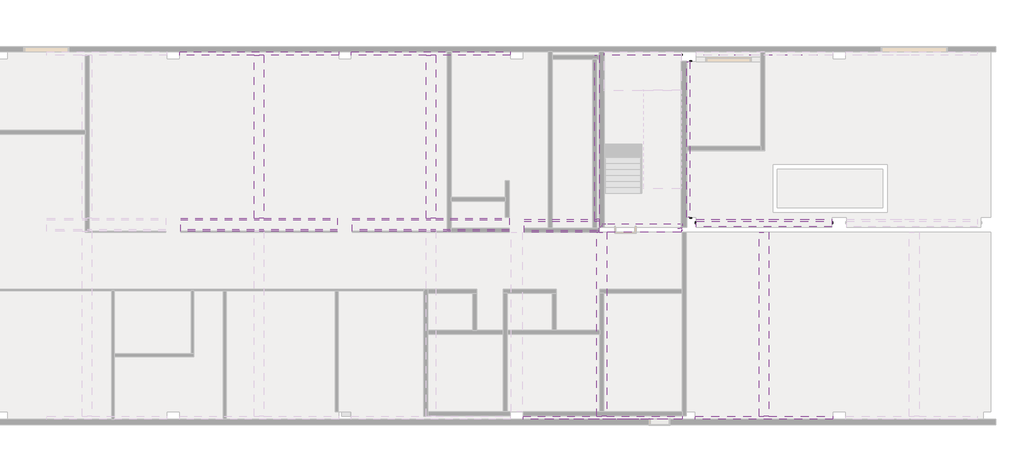
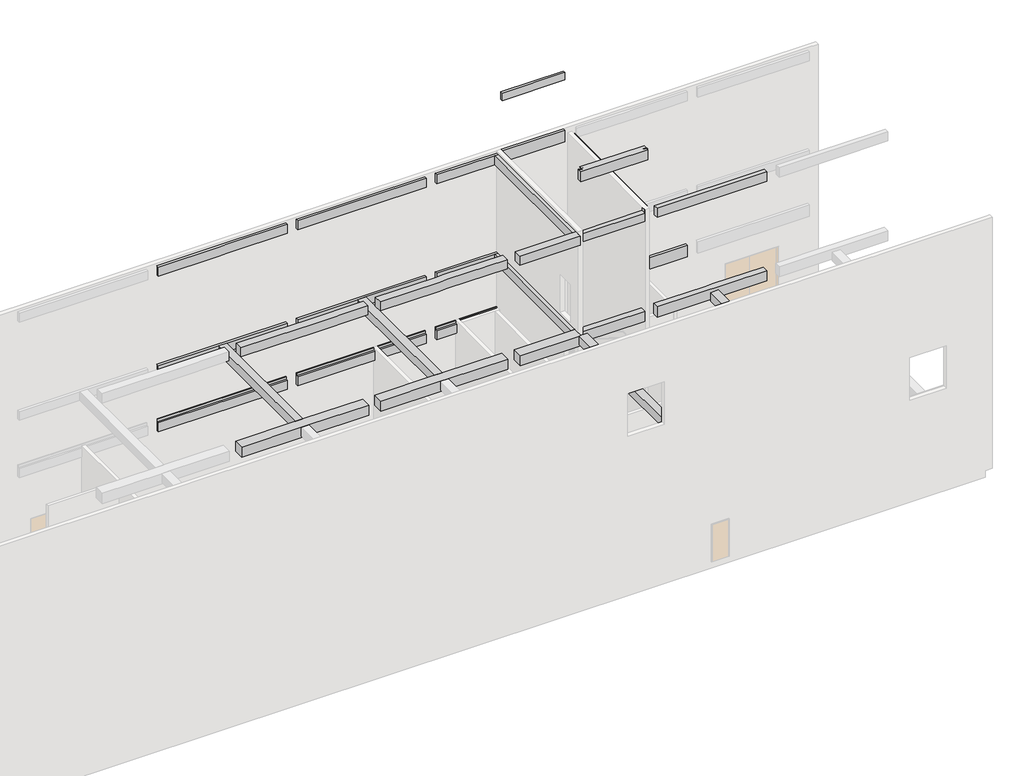
# One storey, part 4 of 5: 55 beams.
"""IFC4 building model written with IfcOpenShell, lengths in millimetres."""

from ifc_helpers import new_model, si_unit, frame, origin, place, context, project, spatial, polyline, outline, extrude, faceted_brep, element, save

model = new_model("IFC4")

# Units and contexts
model_context = context("Model", 3, world=origin())
ifc_project = project(units=[si_unit("LENGTHUNIT", "METRE", prefix="MILLI")], contexts=[model_context])

# Site, building, storey
site = spatial("IfcSite", under=ifc_project)
building = spatial("IfcBuilding", under=site)
storey = spatial("IfcBuildingStorey", under=building, Name="TOC", Elevation=149.9618634)

# Beams
placement = place(None, origin())
element("IfcBeam", 1, ObjectType="RC Beam_Rectangular : H_SB_AR_S16_UG_B500xH700_1G1", at=placement, inside=storey, context=model_context, shape_type="Brep", body=[
    faceted_brep([(61750.0, 799.5208589, -0.0381366), (61750.0, 9149.5208589, -0.0381366), (61750.0, 9149.5208589, -150.0381366), (61750.0, 9149.5208589, -550.0381366), (61750.0, 799.5208589, -550.0381366), (62250.0, 9149.5208589, -550.0381366), (62250.0, 799.5208589, -550.0381366), (62250.0, 9149.5208589, -0.0381366), (62250.0, 799.5208589, -0.0381366), (62250.0, 9149.5208589, -150.0381366)], [[[0, 1, 2, 3, 4]], [[3, 5, 6, 4]], [[7, 8, 6, 5, 9]], [[1, 0, 8, 7]], [[5, 3, 2, 1, 7, 9]], [[4, 6, 8, 0]]]),
])
element("IfcBeam", 2, ObjectType="RC Beam_Rectangular : H_SB_AR_S16_UG_B500xH700_1G1", at=placement, inside=storey, context=model_context, shape_type="Brep", body=[
    faceted_brep([(54700.0, 799.5208589, -0.0381366), (54700.0, 9149.5208589, -0.0381366), (54700.0, 9149.5208589, -150.0381366), (54700.0, 9149.5208589, -550.0381366), (54700.0, 799.5208589, -550.0381366), (54700.0, 799.5208589, -150.0381366), (55200.0, 799.5208589, -550.0381366), (54850.0, 9149.5208589, -550.0381366), (55200.0, 9149.5208589, -550.0381366), (55200.0, 9149.5208589, -0.0381366), (55200.0, 799.5208589, -0.0381366), (55200.0, 9149.5208589, -150.0381366)], [[[0, 1, 2, 3, 4, 5]], [[6, 4, 3, 7, 8]], [[9, 10, 6, 8, 11]], [[1, 0, 10, 9]], [[1, 9, 11, 8, 7, 3, 2]], [[4, 6, 10, 0, 5]]]),
])
element("IfcBeam", 3, ObjectType="RC Beam_Rectangular : H_SB_AR_S16_UG_B450xH700_1B2", at=placement, inside=storey, context=model_context, shape_type="SweptSolid", body=[
    extrude(outline(polyline([(57725.0, 599.5208589), (57275.0, 599.5208589), (57275.0, 9149.5208589), (57725.0, 9149.5208589), (57725.0, 599.5208589)])), frame((0.0, 0.0, -550.0381366), z_axis=(0.0, 0.0, 1.0), x_axis=(1.0, 0.0, 0.0)), (0.0, 0.0, 1.0), 550.0),
])
element("IfcBeam", 4, ObjectType="RC Beam_Rectangular : H_SB_AR_S16_UG_B450xH700_1B2", at=placement, inside=storey, context=model_context, shape_type="SweptSolid", body=[
    extrude(outline(polyline([(60225.0, 599.5208589), (59775.0, 599.5208589), (59775.0, 9149.5208589), (60225.0, 9149.5208589), (60225.0, 599.5208589)])), frame((0.0, 0.0, -550.0381366), z_axis=(0.0, 0.0, 1.0), x_axis=(1.0, 0.0, 0.0)), (0.0, 0.0, 1.0), 550.0),
])
element("IfcBeam", 5, ObjectType="RC Beam_Rectangular : H_SB_AR_S16_UG_B450xH700_1B1A", at=placement, inside=storey, context=model_context, shape_type="Brep", body=[
    faceted_brep([(51175.0, 599.5208589, -0.0381366), (51175.0, 599.5208589, -550.0381366), (51175.0, 9149.5208589, -550.0381366), (51175.0, 9149.5208589, -0.0381366), (50725.0, 599.5208589, -550.0381366), (50725.0, 9199.5208589, -550.0381366), (50725.0, 9799.5208589, -550.0381366), (50825.0, 9799.5208589, -550.0381366), (50825.0, 9149.5208589, -550.0381366), (50725.0, 599.5208589, -0.0381366), (50725.0, 9199.5208589, -0.0381366), (50725.0, 9799.5208589, -0.0381366), (50825.0, 9149.5208589, -0.0381366), (50825.0, 9799.5208589, -0.0381366)], [[[0, 1, 2, 3]], [[4, 5, 6, 7, 8, 2, 1]], [[6, 5, 4, 9, 10, 11]], [[4, 1, 0, 9]], [[0, 3, 12, 13, 11, 10, 9]], [[12, 8, 7, 13]], [[6, 11, 13, 7]], [[8, 12, 3, 2]]]),
])
element("IfcBeam", 6, ObjectType="RC Beam_Rectangular : H_SB_AR_S16_UG_B500xH700_1G3", at=placement, inside=storey, context=model_context, shape_type="SweptSolid", body=[
    extrude(outline(polyline([(-550.0381366, 55300.0), (-550.0381366, 61700.0), (-150.0381366, 61700.0), (-150.0381366, 61650.0), (-0.0381366, 61650.0), (-0.0381366, 55350.0), (-150.0381366, 55350.0), (-150.0381366, 55300.0), (-550.0381366, 55300.0)])), frame((0.0, 9549.5208589, 0.0), z_axis=(0.0, 1.0, 0.0), x_axis=(0.0, 0.0, 1.0)), (0.0, 0.0, 1.0), 100.0),
])
element("IfcBeam", 7, ObjectType="RC Beam_Rectangular : H_SB_AR_S16_UG_B600xH800_1G2", at=placement, inside=storey, context=model_context, shape_type="SweptSolid", body=[
    extrude(outline(polyline([(51225.0, 9799.5208589), (54650.0, 9799.5208589), (54650.0, 9549.5208589), (51225.0, 9549.5208589), (51225.0, 9799.5208589)])), frame((0.0, 0.0, -550.0381366), z_axis=(0.0, 0.0, 1.0), x_axis=(1.0, 0.0, 0.0)), (0.0, 0.0, 1.0), 500.0),
    extrude(outline(polyline([(-150.0381366, 47300.0), (-550.0381366, 47300.0), (-550.0381366, 48250.0), (-650.0381366, 48250.0), (-650.0381366, 49775.0), (-550.0381366, 49775.0), (-550.0381366, 50725.0), (-0.0381366, 50725.0), (-0.0381366, 47350.0), (-150.0381366, 47350.0), (-150.0381366, 47300.0)])), frame((0.0, 9199.5208589, 0.0), z_axis=(0.0, 1.0, 0.0), x_axis=(0.0, 0.0, 1.0)), (0.0, 0.0, 1.0), 600.0),
])
element("IfcBeam", 8, ObjectType="RC Beam_Rectangular : H_SB_AR_S16_UG_B600xH800_1G2", at=placement, inside=storey, context=model_context, shape_type="Brep", body=[
    faceted_brep([(39300.0, 9749.5208589, -550.0381366), (39300.0, 9749.5208589, -150.0381366), (39350.0, 9749.5208589, -150.0381366), (39350.0, 9749.5208589, -0.0381366), (42775.0, 9749.5208589, -0.0381366), (43225.0, 9749.5208589, -0.0381366), (46650.0, 9749.5208589, -0.0381366), (46650.0, 9749.5208589, -150.0381366), (46700.0, 9749.5208589, -150.0381366), (46700.0, 9749.5208589, -550.0381366), (45750.0, 9749.5208589, -550.0381366), (45750.0, 9749.5208589, -650.0381366), (40250.0, 9749.5208589, -650.0381366), (40250.0, 9749.5208589, -550.0381366), (40250.0, 9149.5208589, -650.0381366), (45750.0, 9149.5208589, -650.0381366), (38750.0, 9149.5208589, -550.0381366), (40250.0, 9149.5208589, -550.0381366), (45750.0, 9149.5208589, -550.0381366), (46750.0, 9149.5208589, -550.0381366), (47250.0, 9149.5208589, -550.0381366), (47250.0, 9149.5208589, -150.0381366), (46650.0, 9149.5208589, -150.0381366), (46650.0, 9149.5208589, -0.0381366), (43225.0, 9149.5208589, -0.0381366), (42775.0, 9149.5208589, -0.0381366), (39350.0, 9149.5208589, -0.0381366), (39350.0, 9149.5208589, -150.0381366), (38750.0, 9149.5208589, -150.0381366), (39300.0, 9199.5208589, -550.0381366), (39300.0, 9199.5208589, -150.0381366), (46700.0, 9199.5208589, -150.0381366), (46700.0, 9199.5208589, -550.0381366), (38750.0, 9199.5208589, -550.0381366), (46750.0, 9199.5208589, -550.0381366), (47250.0, 9199.5208589, -550.0381366), (38750.0, 9199.5208589, -150.0381366), (46750.0, 9199.5208589, -150.0381366), (47250.0, 9199.5208589, -150.0381366)], [[[0, 1, 2, 3, 4, 5, 6, 7, 8, 9, 10, 11, 12, 13]], [[14, 12, 11, 15]], [[16, 17, 14, 15, 18, 19, 20, 21, 22, 23, 24, 25, 26, 27, 28]], [[29, 30, 1, 0]], [[31, 32, 9, 8]], [[13, 17, 16, 33, 29, 0]], [[17, 13, 12, 14]], [[18, 10, 9, 32, 34, 35, 20, 19]], [[10, 18, 15, 11]], [[3, 26, 25, 24, 23, 6, 5, 4]], [[30, 29, 33, 36]], [[32, 31, 37, 38, 35, 34]], [[27, 2, 1, 30, 36, 28]], [[2, 27, 26, 3]], [[7, 22, 21, 38, 37, 31, 8]], [[22, 7, 6, 23]], [[36, 33, 16, 28]], [[20, 35, 38, 21]]]),
])
element("IfcBeam", 9, ObjectType="RC Beam_Rectangular : H_SB_AR_S16_UG_B600xH800_1G2", at=placement, inside=storey, context=model_context, shape_type="Brep", body=[
    faceted_brep([(38700.0, 9749.5208589, -150.0381366), (38700.0, 9749.5208589, -550.0381366), (37797.3745649, 9749.5208589, -550.0381366), (37797.3745649, 9749.5208589, -0.0381366), (38650.0, 9749.5208589, -0.0381366), (38650.0, 9749.5208589, -150.0381366), (37797.3745649, 9500.8571094, -550.0381366), (37797.3745649, 9500.8571094, -0.0381366), (38650.0, 9499.9097478, -0.0381366), (38650.0, 9499.9097478, -150.0381366), (38700.0, 9499.8541922, -150.0381366), (38700.0, 9499.8541922, -550.0381366)], [[[0, 1, 2, 3, 4, 5]], [[2, 6, 7, 3]], [[3, 7, 8, 4]], [[5, 9, 10, 0]], [[11, 10, 9, 8, 7, 6]], [[1, 0, 10, 11]], [[2, 1, 11, 6]], [[9, 5, 4, 8]]]),
    faceted_brep([(38749.6109568, 9149.5208589, -150.0381366), (38749.6109568, 9149.5208589, -550.0381366), (38750.0, 9149.5208589, -550.0381366), (38750.0, 9149.5208589, -150.0381366), (38749.6665123, 9199.5208589, -550.0381366), (38750.0, 9199.5208589, -550.0381366), (38749.6665123, 9199.5208589, -150.0381366), (38750.0, 9199.5208589, -150.0381366)], [[[0, 1, 2, 3]], [[1, 4, 5, 2]], [[4, 6, 7, 5]], [[6, 4, 1, 0]], [[3, 2, 5, 7]], [[6, 0, 3, 7]]]),
])
element("IfcBeam", 10, ObjectType="RC Beam_Rectangular : H_SB_AR_S16_UG_B450xH700_1B1", at=placement, inside=storey, context=model_context, shape_type="SweptSolid", body=[
    extrude(outline(polyline([(34775.0, 17399.5208589), (35225.0, 17399.5208589), (35225.0, 9749.5208589), (34775.0, 9749.5208589), (34775.0, 17399.5208589)])), frame((0.0, 0.0, -550.0381366), z_axis=(0.0, 0.0, 1.0), x_axis=(1.0, 0.0, 0.0)), (0.0, 0.0, 1.0), 550.0),
])
element("IfcBeam", 11, ObjectType="RC Beam_Rectangular : H_SB_AR_S16_UG_B450xH700_1B1", at=placement, inside=storey, context=model_context, shape_type="SweptSolid", body=[
    extrude(outline(polyline([(42775.0, 17399.5208589), (43225.0, 17399.5208589), (43225.0, 9749.5208589), (42775.0, 9749.5208589), (42775.0, 17399.5208589)])), frame((0.0, 0.0, -550.0381366), z_axis=(0.0, 0.0, 1.0), x_axis=(1.0, 0.0, 0.0)), (0.0, 0.0, 1.0), 550.0),
])
element("IfcBeam", 12, ObjectType="RC Beam_Rectangular : H_SB_AR_S16_UG_B500xH700_1G1", at=placement, inside=storey, context=model_context, shape_type="SweptSolid", body=[
    extrude(outline(polyline([(17199.5208589, -550.0381366), (9799.5208589, -550.0381366), (9799.5208589, -150.0381366), (9849.5208589, -150.0381366), (9849.5208589, -0.0381366), (17199.5208589, -0.0381366), (17199.5208589, -550.0381366)])), frame((46750.0, 0.0, 0.0), z_axis=(1.0, 0.0, 0.0), x_axis=(0.0, 1.0, 0.0)), (0.0, 0.0, 1.0), 500.0),
])
element("IfcBeam", 13, ObjectType="RC Beam_Rectangular : H_SB_AR_S16_UG_B500xH700_1G1", at=placement, inside=storey, context=model_context, shape_type="SweptSolid", body=[
    extrude(outline(polyline([(9799.5208589, -550.0381366), (9799.5208589, -150.0381366), (9849.5208589, -150.0381366), (9849.5208589, -0.0381366), (17199.5208589, -0.0381366), (17199.5208589, -550.0381366), (9799.5208589, -550.0381366)])), frame((38750.0, 0.0, 0.0), z_axis=(1.0, 0.0, 0.0), x_axis=(0.0, 1.0, 0.0)), (0.0, 0.0, 1.0), 500.0),
])
element("IfcBeam", 14, ObjectType="RC Beam_Rectangular : H_SB_AR_S16_UG_B500xH700_1G1", at=placement, inside=storey, context=model_context, shape_type="SweptSolid", body=[
    extrude(outline(polyline([(17149.5208589, -550.0381366), (9799.5208589, -550.0381366), (9799.5208589, -150.0381366), (9849.5208589, -150.0381366), (9849.5208589, -0.0381366), (17099.5208589, -0.0381366), (17099.5208589, -150.0381366), (17149.5208589, -150.0381366), (17149.5208589, -550.0381366)])), frame((55050.0, 0.0, 0.0), z_axis=(1.0, 0.0, 0.0), x_axis=(0.0, 1.0, 0.0)), (0.0, 0.0, 1.0), 100.0),
    extrude(outline(polyline([(54650.0, 17449.5208589), (54700.0, 17449.5208589), (54700.0, 17399.5208589), (54650.0, 17399.5208589), (54650.0, 17449.5208589)])), frame((0.0, 0.0, -550.0381366), z_axis=(0.0, 0.0, 1.0), x_axis=(1.0, 0.0, 0.0)), (0.0, 0.0, 1.0), 400.0),
])
element("IfcBeam", 15, ObjectType="RC Beam_Rectangular : H_SB_AR_S16_AG_B400xH700_3WG1", at=placement, inside=storey, context=model_context, shape_type="Brep", body=[
    faceted_brep([(31300.0, 17499.5208589, 5949.9618634), (38700.0, 17499.5208589, 5949.9618634), (38700.0, 17549.5208589, 5949.9618634), (31300.0, 17549.5208589, 5949.9618634), (31300.0, 17399.5208589, 5799.9618634), (31300.0, 17399.5208589, 5249.9618634), (34775.0, 17399.5208589, 5249.9618634), (35225.0, 17399.5208589, 5249.9618634), (38700.0, 17399.5208589, 5249.9618634), (38700.0, 17399.5208589, 5799.9618634), (35225.0, 17399.5208589, 5799.9618634), (34775.0, 17399.5208589, 5799.9618634), (31300.0, 17549.5208589, 5249.9618634), (38700.0, 17549.5208589, 5249.9618634), (31300.0, 17499.5208589, 5799.9618634), (38700.0, 17499.5208589, 5799.9618634)], [[[0, 1, 2, 3]], [[4, 5, 6, 7, 8, 9, 10, 11]], [[8, 7, 6, 5, 12, 13]], [[14, 4, 11, 10, 9, 15]], [[0, 14, 15, 1]], [[5, 4, 14, 0, 3, 12]], [[9, 8, 13, 2, 1, 15]], [[3, 2, 13, 12]]]),
])
element("IfcBeam", 16, ObjectType="RC Beam_Rectangular : H_SB_AR_S16_AG_B400xH700_3WG1", at=placement, inside=storey, context=model_context, shape_type="Brep", body=[
    faceted_brep([(39300.0, 17499.5208589, 5949.9618634), (46700.0, 17499.5208589, 5949.9618634), (46700.0, 17549.5208589, 5949.9618634), (39300.0, 17549.5208589, 5949.9618634), (39300.0, 17399.5208589, 5799.9618634), (39300.0, 17399.5208589, 5249.9618634), (42775.0, 17399.5208589, 5249.9618634), (43225.0, 17399.5208589, 5249.9618634), (46700.0, 17399.5208589, 5249.9618634), (46700.0, 17399.5208589, 5799.9618634), (43225.0, 17399.5208589, 5799.9618634), (42775.0, 17399.5208589, 5799.9618634), (39300.0, 17549.5208589, 5249.9618634), (46700.0, 17549.5208589, 5249.9618634), (39300.0, 17499.5208589, 5799.9618634), (46700.0, 17499.5208589, 5799.9618634)], [[[0, 1, 2, 3]], [[4, 5, 6, 7, 8, 9, 10, 11]], [[8, 7, 6, 5, 12, 13]], [[14, 4, 11, 10, 9, 15]], [[0, 14, 15, 1]], [[5, 4, 14, 0, 3, 12]], [[9, 8, 13, 2, 1, 15]], [[3, 2, 13, 12]]]),
])
element("IfcBeam", 17, ObjectType="RC Beam_Rectangular : H_SB_AR_S16_AG_B400xH700_3WG1", at=placement, inside=storey, context=model_context, shape_type="Brep", body=[
    faceted_brep([(51075.0, 17549.5208589, 5949.9618634), (51075.0, 17399.5208589, 5949.9618634), (54650.0, 17399.5208589, 5949.9618634), (54650.0, 17549.5208589, 5949.9618634), (51075.0, 17399.5208589, 5249.9618634), (54650.0, 17399.5208589, 5249.9618634), (51075.0, 17549.5208589, 5249.9618634), (54650.0, 17549.5208589, 5249.9618634)], [[[0, 1, 2, 3]], [[1, 4, 5, 2]], [[4, 6, 7, 5]], [[4, 1, 0, 6]], [[2, 5, 7, 3]], [[0, 3, 7, 6]]]),
    faceted_brep([(50825.0, 17399.5208589, 5249.9618634), (50825.0, 17549.5208589, 5249.9618634), (50825.0, 17549.5208589, 5949.9618634), (50825.0, 17499.5208589, 5949.9618634), (50825.0, 17499.5208589, 5799.9618634), (50825.0, 17399.5208589, 5799.9618634), (50625.0, 17399.5208589, 5799.9618634), (47300.0, 17399.5208589, 5799.9618634), (47300.0, 17399.5208589, 5249.9618634), (50625.0, 17399.5208589, 5249.9618634), (47300.0, 17499.5208589, 5799.9618634), (47300.0, 17499.5208589, 5949.9618634), (47300.0, 17549.5208589, 5949.9618634), (47300.0, 17549.5208589, 5249.9618634)], [[[0, 1, 2, 3, 4, 5]], [[0, 5, 6, 7, 8, 9]], [[5, 4, 10, 7, 6]], [[4, 3, 11, 10]], [[7, 10, 11, 12, 13, 8]], [[12, 2, 1, 13]], [[3, 2, 12, 11]], [[1, 0, 9, 8, 13]]]),
])
element("IfcBeam", 18, ObjectType="RC Beam_Rectangular : H_SB_AR_S16_AG_B400xH700_3WG1", at=placement, inside=storey, context=model_context, shape_type="SweptSolid", body=[
    extrude(outline(polyline([(61700.0, 17399.5208589), (55350.0, 17399.5208589), (55350.0, 17549.5208589), (61700.0, 17549.5208589), (61700.0, 17399.5208589)])), frame((0.0, 0.0, 5249.9618634), z_axis=(0.0, 0.0, 1.0), x_axis=(1.0, 0.0, 0.0)), (0.0, 0.0, 1.0), 700.0),
])
element("IfcBeam", 19, ObjectType="RC Beam_Rectangular : H_SB_AR_S16_AG_B400xH700_3WG1", at=placement, inside=storey, context=model_context, shape_type="Brep", body=[
    faceted_brep([(54700.0, 499.5208589, 5949.9618634), (50950.0, 499.5208589, 5949.9618634), (47300.0, 499.5208589, 5949.9618634), (47300.0, 449.5208589, 5949.9618634), (54700.0, 449.5208589, 5949.9618634), (54700.0, 599.5208589, 5249.9618634), (54700.0, 449.5208589, 5249.9618634), (47300.0, 449.5208589, 5249.9618634), (47300.0, 599.5208589, 5249.9618634), (50725.0, 599.5208589, 5249.9618634), (51175.0, 599.5208589, 5249.9618634), (54700.0, 599.5208589, 5799.9618634), (47300.0, 599.5208589, 5799.9618634), (50725.0, 599.5208589, 5799.9618634), (51175.0, 599.5208589, 5799.9618634), (50950.0, 499.5208589, 5799.9618634), (54700.0, 499.5208589, 5799.9618634), (47300.0, 499.5208589, 5799.9618634)], [[[0, 1, 2, 3, 4]], [[5, 6, 7, 8, 9, 10]], [[11, 5, 10, 9, 8, 12, 13, 14]], [[6, 4, 3, 7]], [[15, 16, 11, 14, 13, 12, 17]], [[15, 1, 0, 16]], [[1, 15, 17, 2]], [[0, 4, 6, 5, 11, 16]], [[3, 2, 17, 12, 8, 7]]]),
])
element("IfcBeam", 20, ObjectType="RC Beam_Rectangular : H_SB_AR_S16_AG_B400xH700_3WG1", at=placement, inside=storey, context=model_context, shape_type="Brep", body=[
    faceted_brep([(61700.0, 449.5208589, 5949.9618634), (61700.0, 499.5208589, 5949.9618634), (55300.0, 499.5208589, 5949.9618634), (55300.0, 449.5208589, 5949.9618634), (61700.0, 599.5208589, 5249.9618634), (61700.0, 449.5208589, 5249.9618634), (55300.0, 449.5208589, 5249.9618634), (55300.0, 599.5208589, 5249.9618634), (58275.0, 599.5208589, 5249.9618634), (58725.0, 599.5208589, 5249.9618634), (61700.0, 599.5208589, 5799.9618634), (55300.0, 599.5208589, 5799.9618634), (58275.0, 599.5208589, 5799.9618634), (58725.0, 599.5208589, 5799.9618634), (61700.0, 499.5208589, 5799.9618634), (55300.0, 499.5208589, 5799.9618634)], [[[0, 1, 2, 3]], [[4, 5, 6, 7, 8, 9]], [[10, 4, 9, 8, 7, 11, 12, 13]], [[5, 0, 3, 6]], [[14, 10, 13, 12, 11, 15]], [[1, 14, 15, 2]], [[1, 0, 5, 4, 10, 14]], [[3, 2, 15, 11, 7, 6]]]),
])
element("IfcBeam", 21, ObjectType="RC Beam_Rectangular : H_SB_AR_S16_AG_B600xH800_3G2", at=placement, inside=storey, context=model_context, shape_type="Brep", body=[
    faceted_brep([(31350.0, 9199.5208589, 5149.9618634), (38650.0, 9199.5208589, 5149.9618634), (38650.0, 9199.5208589, 5799.9618634), (35235.0, 9199.5208589, 5799.9618634), (34785.0, 9199.5208589, 5799.9618634), (31350.0, 9199.5208589, 5799.9618634), (31350.0, 9799.5208589, 5149.9618634), (38650.0, 9799.5208589, 5149.9618634), (31350.0, 9799.5208589, 5799.9618634), (34775.0, 9799.5208589, 5799.9618634), (35225.0, 9799.5208589, 5799.9618634), (38650.0, 9799.5208589, 5799.9618634)], [[[0, 1, 2, 3, 4, 5]], [[1, 0, 6, 7]], [[7, 6, 8, 9, 10, 11]], [[5, 4, 3, 2, 11, 10, 9, 8]], [[6, 0, 5, 8]], [[1, 7, 11, 2]]]),
])
element("IfcBeam", 22, ObjectType="RC Beam_Rectangular : H_SB_AR_S16_AG_B600xH800_3G2", at=placement, inside=storey, context=model_context, shape_type="Brep", body=[
    faceted_brep([(39350.0, 9199.5208589, 5149.9618634), (46650.0, 9199.5208589, 5149.9618634), (46650.0, 9199.5208589, 5799.9618634), (43235.0, 9199.5208589, 5799.9618634), (42785.0, 9199.5208589, 5799.9618634), (39350.0, 9199.5208589, 5799.9618634), (39350.0, 9799.5208589, 5149.9618634), (46650.0, 9799.5208589, 5149.9618634), (39350.0, 9799.5208589, 5799.9618634), (42775.0, 9799.5208589, 5799.9618634), (43225.0, 9799.5208589, 5799.9618634), (46650.0, 9799.5208589, 5799.9618634)], [[[0, 1, 2, 3, 4, 5]], [[1, 0, 6, 7]], [[7, 6, 8, 9, 10, 11]], [[5, 4, 3, 2, 11, 10, 9, 8]], [[6, 0, 5, 8]], [[1, 7, 11, 2]]]),
])
element("IfcBeam", 23, ObjectType="RC Beam_Rectangular : H_SB_AR_S16_AG_B600xH800_3WG2", at=placement, inside=storey, context=model_context, shape_type="Brep", body=[
    faceted_brep([(50825.0, 9149.5208589, 5149.9618634), (50825.0, 9149.5208589, 5799.9618634), (50725.0, 9149.5208589, 5799.9618634), (47350.0, 9149.5208589, 5799.9618634), (47350.0, 9149.5208589, 5149.9618634), (50825.0, 9749.5208589, 5149.9618634), (50825.0, 9749.5208589, 5249.9618634), (50825.0, 9749.5208589, 5799.9618634), (50625.0, 9749.5208589, 5799.9618634), (47350.0, 9749.5208589, 5799.9618634), (47350.0, 9749.5208589, 5149.9618634)], [[[0, 1, 2, 3, 4]], [[0, 5, 6, 7, 1]], [[3, 2, 1, 7, 8, 9]], [[10, 4, 3, 9]], [[5, 0, 4, 10]], [[5, 10, 9, 8, 7, 6]]]),
    faceted_brep([(54650.0, 9399.5208589, 5149.9618634), (54650.0, 9749.5208589, 5149.9618634), (54650.0, 9749.5208589, 5749.9618634), (54650.0, 9399.5208589, 5749.9618634), (51075.0, 9399.5208589, 5749.9618634), (51075.0, 9749.5208589, 5749.9618634), (51075.0, 9749.5208589, 5149.9618634), (51075.0, 9399.5208589, 5149.9618634)], [[[0, 1, 2, 3]], [[4, 5, 6, 7]], [[5, 4, 3, 2]], [[1, 0, 7, 6]], [[1, 6, 5, 2]], [[7, 0, 3, 4]]]),
])
element("IfcBeam", 24, ObjectType="RC Beam_Rectangular : H_SB_AR_S16_AG_B600xH800_3WG2", at=placement, inside=storey, context=model_context, shape_type="SweptSolid", body=[
    extrude(outline(polyline([(55350.0, 9399.5208589), (55350.0, 9749.5208589), (61650.0, 9749.5208589), (61650.0, 9399.5208589), (55350.0, 9399.5208589)])), frame((0.0, 0.0, 5149.9618634), z_axis=(0.0, 0.0, 1.0), x_axis=(1.0, 0.0, 0.0)), (0.0, 0.0, 1.0), 800.0),
])
element("IfcBeam", 25, ObjectType="RC Beam_Rectangular : H_SB_AR_S16_AG_B400xH700_3WG3", at=placement, inside=storey, context=model_context, shape_type="SweptSolid", body=[
    extrude(outline(polyline([(55050.0, 9849.5208589), (54900.0, 9849.5208589), (54900.0, 17099.5208589), (55050.0, 17099.5208589), (55050.0, 9849.5208589)])), frame((0.0, 0.0, 5249.9618634), z_axis=(0.0, 0.0, 1.0), x_axis=(1.0, 0.0, 0.0)), (0.0, 0.0, 1.0), 700.0),
])
element("IfcBeam", 26, ObjectType="RC Beam_Rectangular : H_SB_AR_S16_AG_B450xH700_2WB1", at=placement, inside=storey, context=model_context, shape_type="SweptSolid", body=[
    extrude(outline(polyline([(50825.0, 9749.5208589), (50625.0, 9749.5208589), (50625.0, 17399.5208589), (50825.0, 17399.5208589), (50825.0, 9749.5208589)])), frame((0.0, 0.0, 5249.9618634), z_axis=(0.0, 0.0, 1.0), x_axis=(1.0, 0.0, 0.0)), (0.0, 0.0, 1.0), 550.0),
])
element("IfcBeam", 27, ObjectType="RC Beam_Rectangular : H_SB_AR_S16_AG_B450xH700_3B1", at=placement, inside=storey, context=model_context, shape_type="SweptSolid", body=[
    extrude(outline(polyline([(58275.0, 9149.5208589), (58725.0, 9149.5208589), (58725.0, 599.5208589), (58275.0, 599.5208589), (58275.0, 9149.5208589)])), frame((0.0, 0.0, 5249.9618634), z_axis=(0.0, 0.0, 1.0), x_axis=(1.0, 0.0, 0.0)), (0.0, 0.0, 1.0), 550.0),
])
element("IfcBeam", 28, ObjectType="RC Beam_Rectangular : H_SB_AR_S16_AG_B400xH700_3WG1", at=placement, inside=storey, context=model_context, shape_type="Brep", body=[
    faceted_brep([(31300.0, 17399.5208589, 9269.9618634), (31300.0, 17399.5208589, 8749.9618634), (34775.0, 17399.5208589, 8749.9618634), (35225.0, 17399.5208589, 8749.9618634), (38700.0, 17399.5208589, 8749.9618634), (38700.0, 17399.5208589, 9269.9618634), (35225.0, 17399.5208589, 9269.9618634), (34775.0, 17399.5208589, 9269.9618634), (31300.0, 17549.5208589, 8749.9618634), (38700.0, 17549.5208589, 8749.9618634), (31300.0, 17549.5208589, 9269.9618634), (38700.0, 17549.5208589, 9269.9618634)], [[[0, 1, 2, 3, 4, 5, 6, 7]], [[4, 3, 2, 1, 8, 9]], [[10, 0, 7, 6, 5, 11]], [[1, 0, 10, 8]], [[5, 4, 9, 11]], [[9, 8, 10, 11]]]),
])
element("IfcBeam", 29, ObjectType="RC Beam_Rectangular : H_SB_AR_S16_AG_B400xH700_3WG1", at=placement, inside=storey, context=model_context, shape_type="Brep", body=[
    faceted_brep([(39300.0, 17399.5208589, 9269.9618634), (39300.0, 17399.5208589, 8749.9618634), (42775.0, 17399.5208589, 8749.9618634), (43225.0, 17399.5208589, 8749.9618634), (46700.0, 17399.5208589, 8749.9618634), (46700.0, 17399.5208589, 9269.9618634), (43225.0, 17399.5208589, 9269.9618634), (42775.0, 17399.5208589, 9269.9618634), (39300.0, 17549.5208589, 8749.9618634), (46700.0, 17549.5208589, 8749.9618634), (39300.0, 17549.5208589, 9269.9618634), (46700.0, 17549.5208589, 9269.9618634)], [[[0, 1, 2, 3, 4, 5, 6, 7]], [[4, 3, 2, 1, 8, 9]], [[10, 0, 7, 6, 5, 11]], [[1, 0, 10, 8]], [[5, 4, 9, 11]], [[9, 8, 10, 11]]]),
])
element("IfcBeam", 30, ObjectType="RC Beam_Rectangular : H_SB_AR_S16_AG_B400xH700_3WG1", at=placement, inside=storey, context=model_context, shape_type="Brep", body=[
    faceted_brep([(51075.0, 17549.5208589, 9449.9618634), (51075.0, 17399.5208589, 9449.9618634), (54650.0, 17399.5208589, 9449.9618634), (54650.0, 17549.5208589, 9449.9618634), (51075.0, 17399.5208589, 9269.9618634), (51075.0, 17399.5208589, 8749.9618634), (54650.0, 17399.5208589, 8749.9618634), (51075.0, 17549.5208589, 8749.9618634), (54650.0, 17549.5208589, 8749.9618634), (51075.0, 17549.5208589, 9269.9618634)], [[[0, 1, 2, 3]], [[1, 4, 5, 6, 2]], [[5, 7, 8, 6]], [[7, 5, 4, 1, 0, 9]], [[2, 6, 8, 3]], [[0, 3, 8, 7, 9]]]),
    faceted_brep([(50825.0, 17399.5208589, 8749.9618634), (50825.0, 17549.5208589, 8749.9618634), (50825.0, 17549.5208589, 9269.9618634), (50825.0, 17399.5208589, 9269.9618634), (50625.0, 17399.5208589, 9269.9618634), (47300.0, 17399.5208589, 9269.9618634), (47300.0, 17399.5208589, 8749.9618634), (50625.0, 17399.5208589, 8749.9618634), (47300.0, 17549.5208589, 9269.9618634), (47300.0, 17549.5208589, 8749.9618634)], [[[0, 1, 2, 3]], [[0, 3, 4, 5, 6, 7]], [[3, 2, 8, 5, 4]], [[5, 8, 9, 6]], [[1, 9, 8, 2]], [[1, 0, 7, 6, 9]]]),
])
element("IfcBeam", 31, ObjectType="RC Beam_Rectangular : H_SB_AR_S16_AG_B400xH700_3WG1", at=placement, inside=storey, context=model_context, shape_type="Brep", body=[
    faceted_brep([(54700.0, 599.5208589, 8749.9618634), (54700.0, 449.5208589, 8749.9618634), (47300.0, 449.5208589, 8749.9618634), (47300.0, 599.5208589, 8749.9618634), (50725.0, 599.5208589, 8749.9618634), (51175.0, 599.5208589, 8749.9618634), (54700.0, 599.5208589, 9269.9618634), (47300.0, 599.5208589, 9269.9618634), (50725.0, 599.5208589, 9269.9618634), (51175.0, 599.5208589, 9269.9618634), (54700.0, 449.5208589, 9269.9618634), (50825.0, 449.5208589, 9269.9618634), (47300.0, 449.5208589, 9269.9618634)], [[[0, 1, 2, 3, 4, 5]], [[6, 0, 5, 4, 3, 7, 8, 9]], [[1, 10, 11, 12, 2]], [[10, 6, 9, 8, 7, 12, 11]], [[1, 0, 6, 10]], [[3, 2, 12, 7]]]),
])
element("IfcBeam", 32, ObjectType="RC Beam_Rectangular : H_SB_AR_S16_AG_B400xH700_3WG1", at=placement, inside=storey, context=model_context, shape_type="Brep", body=[
    faceted_brep([(61700.0, 599.5208589, 8749.9618634), (61700.0, 449.5208589, 8749.9618634), (55300.0, 449.5208589, 8749.9618634), (55300.0, 599.5208589, 8749.9618634), (58275.0, 599.5208589, 8749.9618634), (58725.0, 599.5208589, 8749.9618634), (61700.0, 599.5208589, 9269.9618634), (55300.0, 599.5208589, 9269.9618634), (58275.0, 599.5208589, 9269.9618634), (58725.0, 599.5208589, 9269.9618634), (61700.0, 449.5208589, 9269.9618634), (55300.0, 449.5208589, 9269.9618634)], [[[0, 1, 2, 3, 4, 5]], [[6, 0, 5, 4, 3, 7, 8, 9]], [[1, 10, 11, 2]], [[10, 6, 9, 8, 7, 11]], [[1, 0, 6, 10]], [[3, 2, 11, 7]]]),
])
element("IfcBeam", 33, ObjectType="RC Beam_Rectangular : H_SB_AR_S16_AG_B600xH800_3G2", at=placement, inside=storey, context=model_context, shape_type="Brep", body=[
    faceted_brep([(31350.0, 9199.5208589, 8649.9618634), (38650.0, 9199.5208589, 8649.9618634), (38650.0, 9199.5208589, 9269.9618634), (35225.0, 9199.5208589, 9269.9618634), (34775.0, 9199.5208589, 9269.9618634), (31350.0, 9199.5208589, 9269.9618634), (31350.0, 9799.5208589, 8649.9618634), (38650.0, 9799.5208589, 8649.9618634), (31350.0, 9799.5208589, 9269.9618634), (34775.0, 9799.5208589, 9269.9618634), (35225.0, 9799.5208589, 9269.9618634), (38650.0, 9799.5208589, 9269.9618634)], [[[0, 1, 2, 3, 4, 5]], [[1, 0, 6, 7]], [[7, 6, 8, 9, 10, 11]], [[5, 4, 3, 2, 11, 10, 9, 8]], [[6, 0, 5, 8]], [[1, 7, 11, 2]]]),
])
element("IfcBeam", 34, ObjectType="RC Beam_Rectangular : H_SB_AR_S16_AG_B600xH800_3G2", at=placement, inside=storey, context=model_context, shape_type="Brep", body=[
    faceted_brep([(39350.0, 9199.5208589, 8649.9618634), (46650.0, 9199.5208589, 8649.9618634), (46650.0, 9199.5208589, 9269.9618634), (43225.0, 9199.5208589, 9269.9618634), (42775.0, 9199.5208589, 9269.9618634), (39350.0, 9199.5208589, 9269.9618634), (39350.0, 9799.5208589, 8649.9618634), (46650.0, 9799.5208589, 8649.9618634), (39350.0, 9799.5208589, 9269.9618634), (42775.0, 9799.5208589, 9269.9618634), (43225.0, 9799.5208589, 9269.9618634), (46650.0, 9799.5208589, 9269.9618634)], [[[0, 1, 2, 3, 4, 5]], [[1, 0, 6, 7]], [[7, 6, 8, 9, 10, 11]], [[5, 4, 3, 2, 11, 10, 9, 8]], [[6, 0, 5, 8]], [[1, 7, 11, 2]]]),
])
element("IfcBeam", 35, ObjectType="RC Beam_Rectangular : H_SB_AR_S16_AG_B600xH800_3WG2", at=placement, inside=storey, context=model_context, shape_type="Brep", body=[
    faceted_brep([(50825.0, 9149.5208589, 8649.9618634), (50825.0, 9149.5208589, 9269.9618634), (50725.0, 9149.5208589, 9269.9618634), (47350.0, 9149.5208589, 9269.9618634), (47350.0, 9149.5208589, 8649.9618634), (50825.0, 9749.5208589, 8649.9618634), (50825.0, 9749.5208589, 8749.9618634), (50825.0, 9749.5208589, 9269.9618634), (50625.0, 9749.5208589, 9269.9618634), (47350.0, 9749.5208589, 9269.9618634), (47350.0, 9749.5208589, 8649.9618634)], [[[0, 1, 2, 3, 4]], [[0, 5, 6, 7, 1]], [[3, 2, 1, 7, 8, 9]], [[10, 4, 3, 9]], [[5, 0, 4, 10]], [[5, 10, 9, 8, 7, 6]]]),
    faceted_brep([(54650.0, 9399.5208589, 8649.9618634), (54650.0, 9749.5208589, 8649.9618634), (54650.0, 9749.5208589, 9249.9618634), (54650.0, 9399.5208589, 9249.9618634), (51075.0, 9399.5208589, 9249.9618634), (51075.0, 9749.5208589, 9249.9618634), (51075.0, 9749.5208589, 8649.9618634), (51075.0, 9399.5208589, 8649.9618634)], [[[0, 1, 2, 3]], [[4, 5, 6, 7]], [[5, 4, 3, 2]], [[1, 0, 7, 6]], [[1, 6, 5, 2]], [[7, 0, 3, 4]]]),
])
element("IfcBeam", 36, ObjectType="RC Beam_Rectangular : H_SB_AR_S16_AG_B600xH800_3WG2", at=placement, inside=storey, context=model_context, shape_type="Brep", body=[
    faceted_brep([(55350.0, 9399.5208589, 8649.9618634), (55350.0, 9749.5208589, 8649.9618634), (61650.0, 9749.5208589, 8649.9618634), (61650.0, 9399.5208589, 8649.9618634), (55350.0, 9749.5208589, 9269.9618634), (58275.0, 9749.5208589, 9269.9618634), (58725.0, 9749.5208589, 9269.9618634), (61650.0, 9749.5208589, 9269.9618634), (55350.0, 9399.5208589, 9269.9618634), (61650.0, 9399.5208589, 9269.9618634)], [[[0, 1, 2, 3]], [[1, 4, 5, 6, 7, 2]], [[8, 0, 3, 9]], [[4, 8, 9, 7, 6, 5]], [[1, 0, 8, 4]], [[3, 2, 7, 9]]]),
])
element("IfcBeam", 37, ObjectType="RC Beam_Rectangular : H_SB_AR_S16_AG_B400xH700_3WG3", at=placement, inside=storey, context=model_context, shape_type="SweptSolid", body=[
    extrude(outline(polyline([(54900.0, 17099.5208589), (55050.0, 17099.5208589), (55050.0, 9849.5208589), (54900.0, 9849.5208589), (54900.0, 17099.5208589)])), frame((0.0, 0.0, 8749.9618634), z_axis=(0.0, 0.0, 1.0), x_axis=(1.0, 0.0, 0.0)), (0.0, 0.0, 1.0), 520.0),
])
element("IfcBeam", 38, ObjectType="RC Beam_Rectangular : H_SB_AR_S16_AG_B450xH700_3WB1", at=placement, inside=storey, context=model_context, shape_type="SweptSolid", body=[
    extrude(outline(polyline([(50625.0, 9749.5208589), (50625.0, 17399.5208589), (50825.0, 17399.5208589), (50825.0, 9749.5208589), (50625.0, 9749.5208589)])), frame((0.0, 0.0, 8749.9618634), z_axis=(0.0, 0.0, 1.0), x_axis=(1.0, 0.0, 0.0)), (0.0, 0.0, 1.0), 520.0),
])
element("IfcBeam", 39, ObjectType="RC Beam_Rectangular : H_SB_AR_S16_AG_B450xH700_3B1", at=placement, inside=storey, context=model_context, shape_type="SweptSolid", body=[
    extrude(outline(polyline([(34775.0, 17399.5208589), (35225.0, 17399.5208589), (35225.0, 9799.5208589), (34775.0, 9799.5208589), (34775.0, 17399.5208589)])), frame((0.0, 0.0, 8749.9618634), z_axis=(0.0, 0.0, 1.0), x_axis=(1.0, 0.0, 0.0)), (0.0, 0.0, 1.0), 520.0),
])
element("IfcBeam", 40, ObjectType="RC Beam_Rectangular : H_SB_AR_S16_AG_B450xH700_3B1", at=placement, inside=storey, context=model_context, shape_type="SweptSolid", body=[
    extrude(outline(polyline([(42775.0, 17399.5208589), (43225.0, 17399.5208589), (43225.0, 9799.5208589), (42775.0, 9799.5208589), (42775.0, 17399.5208589)])), frame((0.0, 0.0, 8749.9618634), z_axis=(0.0, 0.0, 1.0), x_axis=(1.0, 0.0, 0.0)), (0.0, 0.0, 1.0), 520.0),
])
element("IfcBeam", 41, ObjectType="RC Beam_Rectangular : H_SB_AR_S16_AG_B450xH700_3B1A", at=placement, inside=storey, context=model_context, shape_type="Brep", body=[
    faceted_brep([(50725.0, 9149.5208589, 8749.9618634), (50725.0, 599.5208589, 8749.9618634), (50725.0, 599.5208589, 9269.9618634), (50725.0, 9149.5208589, 9269.9618634), (51175.0, 9149.5208589, 8749.9618634), (51175.0, 599.5208589, 8749.9618634), (51175.0, 9149.5208589, 9269.9618634), (51175.0, 599.5208589, 9269.9618634), (50825.0, 9149.5208589, 9269.9618634)], [[[0, 1, 2, 3]], [[4, 5, 1, 0]], [[5, 4, 6, 7]], [[4, 0, 3, 8, 6]], [[1, 5, 7, 2]], [[3, 2, 7, 6, 8]]]),
])
element("IfcBeam", 42, ObjectType="RC Beam_Rectangular : H_SB_AR_S16_AG_B450xH700_3B1A", at=placement, inside=storey, context=model_context, shape_type="SweptSolid", body=[
    extrude(outline(polyline([(58275.0, 9149.5208589), (58725.0, 9149.5208589), (58725.0, 599.5208589), (58275.0, 599.5208589), (58275.0, 9149.5208589)])), frame((0.0, 0.0, 8749.9618634), z_axis=(0.0, 0.0, 1.0), x_axis=(1.0, 0.0, 0.0)), (0.0, 0.0, 1.0), 520.0),
])
element("IfcBeam", 43, ObjectType="RC Beam_Rectangular : H_SB_AR_S16_AG_B400xH700_RWG1", at=placement, inside=storey, context=model_context, shape_type="Brep", body=[
    faceted_brep([(31300.0, 17399.5208589, 15259.9618634), (31300.0, 17399.5208589, 14709.9618634), (34775.0, 17399.5208589, 14709.9618634), (35225.0, 17399.5208589, 14709.9618634), (38700.0, 17399.5208589, 14709.9618634), (38700.0, 17399.5208589, 15259.9618634), (35225.0, 17399.5208589, 15259.9618634), (34775.0, 17399.5208589, 15259.9618634), (31300.0, 17549.5208589, 14709.9618634), (38700.0, 17549.5208589, 14709.9618634), (31300.0, 17549.5208589, 15259.9618634), (38700.0, 17549.5208589, 15259.9618634)], [[[0, 1, 2, 3, 4, 5, 6, 7]], [[4, 3, 2, 1, 8, 9]], [[10, 0, 7, 6, 5, 11]], [[1, 0, 10, 8]], [[5, 4, 9, 11]], [[9, 8, 10, 11]]]),
])
element("IfcBeam", 44, ObjectType="RC Beam_Rectangular : H_SB_AR_S16_AG_B400xH700_RWG1", at=placement, inside=storey, context=model_context, shape_type="Brep", body=[
    faceted_brep([(39300.0, 17399.5208589, 15259.9618634), (39300.0, 17399.5208589, 14709.9618634), (42775.0, 17399.5208589, 14709.9618634), (43225.0, 17399.5208589, 14709.9618634), (46700.0, 17399.5208589, 14709.9618634), (46700.0, 17399.5208589, 15259.9618634), (43225.0, 17399.5208589, 15259.9618634), (42775.0, 17399.5208589, 15259.9618634), (39300.0, 17549.5208589, 14709.9618634), (46700.0, 17549.5208589, 14709.9618634), (39300.0, 17549.5208589, 15259.9618634), (46700.0, 17549.5208589, 15259.9618634)], [[[0, 1, 2, 3, 4, 5, 6, 7]], [[4, 3, 2, 1, 8, 9]], [[10, 0, 7, 6, 5, 11]], [[1, 0, 10, 8]], [[5, 4, 9, 11]], [[9, 8, 10, 11]]]),
])
element("IfcBeam", 45, ObjectType="RC Beam_Rectangular : H_SB_AR_S16_AG_B400xH700_RWG1", at=placement, inside=storey, context=model_context, shape_type="Brep", body=[
    faceted_brep([(51075.0, 17549.5208589, 15409.9618634), (51075.0, 17399.5208589, 15409.9618634), (54650.0, 17399.5208589, 15409.9618634), (54650.0, 17549.5208589, 15409.9618634), (51075.0, 17399.5208589, 15259.9618634), (51075.0, 17399.5208589, 14709.9618634), (54650.0, 17399.5208589, 14709.9618634), (51075.0, 17549.5208589, 14709.9618634), (54650.0, 17549.5208589, 14709.9618634), (51075.0, 17549.5208589, 15259.9618634), (54650.0, 17549.5208589, 15259.9618634)], [[[0, 1, 2, 3]], [[1, 4, 5, 6, 2]], [[5, 7, 8, 6]], [[7, 5, 4, 1, 0, 9]], [[2, 6, 8, 10, 3]], [[0, 3, 10, 8, 7, 9]]]),
    faceted_brep([(50825.0, 17399.5208589, 14709.9618634), (50825.0, 17549.5208589, 14709.9618634), (50825.0, 17549.5208589, 15259.9618634), (50825.0, 17399.5208589, 15259.9618634), (50625.0, 17399.5208589, 15259.9618634), (47300.0, 17399.5208589, 15259.9618634), (47300.0, 17399.5208589, 14709.9618634), (50625.0, 17399.5208589, 14709.9618634), (47300.0, 17549.5208589, 15259.9618634), (47300.0, 17549.5208589, 14709.9618634)], [[[0, 1, 2, 3]], [[0, 3, 4, 5, 6, 7]], [[3, 2, 8, 5, 4]], [[5, 8, 9, 6]], [[1, 9, 8, 2]], [[1, 0, 7, 6, 9]]]),
])
element("IfcBeam", 46, ObjectType="RC Beam_Rectangular : H_SB_AR_S16_AG_B400xH700_RWG1", at=placement, inside=storey, context=model_context, shape_type="Brep", body=[
    faceted_brep([(54700.0, 599.5208589, 14709.9618634), (54700.0, 449.5208589, 14709.9618634), (47300.0, 449.5208589, 14709.9618634), (47300.0, 599.5208589, 14709.9618634), (50725.0, 599.5208589, 14709.9618634), (51175.0, 599.5208589, 14709.9618634), (54700.0, 599.5208589, 15259.9618634), (47300.0, 599.5208589, 15259.9618634), (50725.0, 599.5208589, 15259.9618634), (51175.0, 599.5208589, 15259.9618634), (54700.0, 449.5208589, 15259.9618634), (50825.0, 449.5208589, 15259.9618634), (47300.0, 449.5208589, 15259.9618634)], [[[0, 1, 2, 3, 4, 5]], [[6, 0, 5, 4, 3, 7, 8, 9]], [[1, 10, 11, 12, 2]], [[10, 6, 9, 8, 7, 12, 11]], [[1, 0, 6, 10]], [[3, 2, 12, 7]]]),
])
element("IfcBeam", 47, ObjectType="RC Beam_Rectangular : H_SB_AR_S16_AG_B400xH700_RWG1", at=placement, inside=storey, context=model_context, shape_type="Brep", body=[
    faceted_brep([(61700.0, 599.5208589, 14709.9618634), (61700.0, 449.5208589, 14709.9618634), (55300.0, 449.5208589, 14709.9618634), (55300.0, 599.5208589, 14709.9618634), (58275.0, 599.5208589, 14709.9618634), (58725.0, 599.5208589, 14709.9618634), (61700.0, 599.5208589, 15259.9618634), (55300.0, 599.5208589, 15259.9618634), (58275.0, 599.5208589, 15259.9618634), (58725.0, 599.5208589, 15259.9618634), (61700.0, 449.5208589, 15259.9618634), (55300.0, 449.5208589, 15259.9618634)], [[[0, 1, 2, 3, 4, 5]], [[6, 0, 5, 4, 3, 7, 8, 9]], [[1, 10, 11, 2]], [[10, 6, 9, 8, 7, 11]], [[1, 0, 6, 10]], [[3, 2, 11, 7]]]),
])
element("IfcBeam", 48, ObjectType="RC Beam_Rectangular : H_SB_AR_S16_AG_B450xH700_RWG3", at=placement, inside=storey, context=model_context, shape_type="Brep", body=[
    faceted_brep([(55350.0, 9674.5208589, 14709.9618634), (55350.0, 9674.5208589, 15259.9618634), (58275.0, 9674.5208589, 15259.9618634), (58725.0, 9674.5208589, 15259.9618634), (61650.0, 9674.5208589, 15259.9618634), (61650.0, 9674.5208589, 14709.9618634), (58725.0, 9674.5208589, 14709.9618634), (58275.0, 9674.5208589, 14709.9618634), (55350.0, 9399.5208589, 14709.9618634), (61650.0, 9399.5208589, 14709.9618634), (55350.0, 9399.5208589, 15259.9618634), (61650.0, 9399.5208589, 15259.9618634)], [[[0, 1, 2, 3, 4, 5, 6, 7]], [[8, 0, 7, 6, 5, 9]], [[10, 8, 9, 11]], [[1, 10, 11, 4, 3, 2]], [[1, 0, 8, 10]], [[5, 4, 11, 9]]]),
])
element("IfcBeam", 49, ObjectType="RC Beam_Rectangular : H_SB_AR_S16_AG_B450xH700_RWG3", at=placement, inside=storey, context=model_context, shape_type="Brep", body=[
    faceted_brep([(50825.0, 9674.5208589, 15259.9618634), (50825.0, 9674.5208589, 14709.9618634), (50625.0, 9674.5208589, 14709.9618634), (47350.0, 9674.5208589, 14709.9618634), (47350.0, 9674.5208589, 15259.9618634), (50625.0, 9674.5208589, 15259.9618634), (50825.0, 9224.5208589, 14709.9618634), (50725.0, 9224.5208589, 14709.9618634), (47350.0, 9224.5208589, 14709.9618634), (50825.0, 9224.5208589, 15259.9618634), (50725.0, 9224.5208589, 15259.9618634), (47350.0, 9224.5208589, 15259.9618634)], [[[0, 1, 2, 3, 4, 5]], [[1, 6, 7, 8, 3, 2]], [[6, 9, 10, 11, 8, 7]], [[6, 1, 0, 9]], [[9, 0, 5, 4, 11, 10]], [[4, 3, 8, 11]]]),
    faceted_brep([(51075.0, 9674.5208589, 14709.9618634), (51075.0, 9399.5208589, 14709.9618634), (51075.0, 9399.5208589, 15209.9618634), (51075.0, 9674.5208589, 15209.9618634), (54647.235546, 9674.5208589, 15409.9618634), (54647.235546, 9399.5208589, 15409.9618634), (54650.0, 9399.5208589, 15409.9618634), (54650.0, 9674.5208589, 15409.9618634), (54647.235546, 9674.5208589, 15209.9618634), (54650.0, 9674.5208589, 15259.9618634), (54650.0, 9674.5208589, 14709.9618634), (54650.0, 9399.5208589, 14709.9618634), (54650.0, 9399.5208589, 15259.9618634), (54647.235546, 9399.5208589, 15209.9618634)], [[[0, 1, 2, 3]], [[4, 5, 6, 7]], [[0, 3, 8, 4, 7, 9, 10]], [[1, 0, 10, 11]], [[7, 6, 12, 11, 10, 9]], [[13, 8, 3, 2]], [[8, 13, 5, 4]], [[2, 1, 11, 12, 6, 5, 13]]]),
])
element("IfcBeam", 50, ObjectType="RC Beam_Rectangular : H_SB_AR_S16_AG_B400xH700_RWG4", at=placement, inside=storey, context=model_context, shape_type="SweptSolid", body=[
    extrude(outline(polyline([(55050.0, 9849.5208589), (54900.0, 9849.5208589), (54900.0, 17099.5208589), (55050.0, 17099.5208589), (55050.0, 9849.5208589)])), frame((0.0, 0.0, 14709.9618634), z_axis=(0.0, 0.0, 1.0), x_axis=(1.0, 0.0, 0.0)), (0.0, 0.0, 1.0), 550.0),
])
element("IfcBeam", 51, ObjectType="RC Beam_Rectangular : H_SB_AR_S16_AG_B450xH700_RWB1", at=placement, inside=storey, context=model_context, shape_type="SweptSolid", body=[
    extrude(outline(polyline([(50625.0, 9674.5208589), (50625.0, 17399.5208589), (50825.0, 17399.5208589), (50825.0, 9674.5208589), (50625.0, 9674.5208589)])), frame((0.0, 0.0, 14709.9618634), z_axis=(0.0, 0.0, 1.0), x_axis=(1.0, 0.0, 0.0)), (0.0, 0.0, 1.0), 550.0),
])
element("IfcBeam", 52, ObjectType="RC Beam_Rectangular : H_SB_AR_S16_AG_B450xH700_RG2", at=placement, inside=storey, context=model_context, shape_type="Brep", body=[
    faceted_brep([(31350.0, 9274.5208589, 14709.9618634), (34775.0, 9274.5208589, 14709.9618634), (35225.0, 9274.5208589, 14709.9618634), (38650.0, 9274.5208589, 14709.9618634), (38650.0, 9274.5208589, 15259.9618634), (35225.0, 9274.5208589, 15259.9618634), (34775.0, 9274.5208589, 15259.9618634), (31350.0, 9274.5208589, 15259.9618634), (31350.0, 9724.5208589, 14709.9618634), (34775.0, 9724.5208589, 14709.9618634), (35225.0, 9724.5208589, 14709.9618634), (38650.0, 9724.5208589, 14709.9618634), (31350.0, 9724.5208589, 15259.9618634), (34775.0, 9724.5208589, 15259.9618634), (35225.0, 9724.5208589, 15259.9618634), (38650.0, 9724.5208589, 15259.9618634)], [[[0, 1, 2, 3, 4, 5, 6, 7]], [[3, 2, 1, 0, 8, 9, 10, 11]], [[11, 10, 9, 8, 12, 13, 14, 15]], [[7, 6, 5, 4, 15, 14, 13, 12]], [[8, 0, 7, 12]], [[3, 11, 15, 4]]]),
])
element("IfcBeam", 53, ObjectType="RC Beam_Rectangular : H_SB_AR_S16_AG_B450xH700_RG2", at=placement, inside=storey, context=model_context, shape_type="Brep", body=[
    faceted_brep([(39350.0, 9274.5208589, 14709.9618634), (42775.0, 9274.5208589, 14709.9618634), (43225.0, 9274.5208589, 14709.9618634), (46650.0, 9274.5208589, 14709.9618634), (46650.0, 9274.5208589, 15259.9618634), (43225.0, 9274.5208589, 15259.9618634), (42775.0, 9274.5208589, 15259.9618634), (39350.0, 9274.5208589, 15259.9618634), (39350.0, 9724.5208589, 14709.9618634), (42775.0, 9724.5208589, 14709.9618634), (43225.0, 9724.5208589, 14709.9618634), (46650.0, 9724.5208589, 14709.9618634), (39350.0, 9724.5208589, 15259.9618634), (42775.0, 9724.5208589, 15259.9618634), (43225.0, 9724.5208589, 15259.9618634), (46650.0, 9724.5208589, 15259.9618634)], [[[0, 1, 2, 3, 4, 5, 6, 7]], [[3, 2, 1, 0, 8, 9, 10, 11]], [[11, 10, 9, 8, 12, 13, 14, 15]], [[7, 6, 5, 4, 15, 14, 13, 12]], [[8, 0, 7, 12]], [[3, 11, 15, 4]]]),
])
element("IfcBeam", 54, ObjectType="RC Beam_Rectangular : H_SB_AR_S16_AG_B400xH600_PHWG2", at=placement, inside=storey, context=model_context, shape_type="SweptSolid", body=[
    extrude(outline(polyline([(17399.5208589, 18449.9618634), (17399.5208589, 18904.7247473), (17549.5208589, 18901.8504958), (17549.5208589, 18449.9618634), (17399.5208589, 18449.9618634)])), frame((51075.0, 0.0, 0.0), z_axis=(1.0, 0.0, 0.0), x_axis=(0.0, 1.0, 0.0)), (0.0, 0.0, 1.0), 3575.0),
])
element("IfcBeam", 55, ObjectType="RC Beam_Rectangular : H_SB_AR_S16_AG_B400xH600_PHWG2", at=placement, inside=storey, context=model_context, shape_type="Brep", body=[
    faceted_brep([(50975.0, 9549.5208589, 19209.9618634), (50975.0, 9299.5208589, 19209.9618634), (50825.0, 9299.5208589, 19209.9618634), (50825.0, 9149.5208589, 19209.9618634), (54650.0, 9149.5208589, 19209.9618634), (54650.0, 9224.5208589, 19209.9618634), (54700.0, 9224.5208589, 19209.9618634), (54700.0, 9274.5208589, 19209.9618634), (54500.0, 9274.5208589, 19209.9618634), (54500.0, 9349.5208589, 19209.9618634), (54700.0, 9349.5208589, 19209.9618634), (54700.0, 9549.5208589, 19209.9618634), (50825.0, 9149.5208589, 18609.9618634), (54650.0, 9149.5208589, 18609.9618634), (50825.0, 9399.5208589, 18609.9618634), (51075.0, 9399.5208589, 18609.9618634), (51075.0, 9549.5208589, 18609.9618634), (51225.0, 9549.5208589, 18609.9618634), (54500.0, 9549.5208589, 18609.9618634), (54500.0, 9343.7032241, 18609.9618634), (54650.0, 9343.7032241, 18609.9618634), (54700.0, 9549.5208589, 19206.0830755), (54500.0, 9549.5208589, 19206.0830755), (51075.0, 9549.5208589, 19203.8442163), (50975.0, 9549.5208589, 19203.8442163), (50975.0, 9299.5208589, 19208.5500987), (50975.0, 9399.5208589, 19206.6677457), (50825.0, 9299.5208589, 19208.5500987), (50825.0, 9399.5208589, 19206.6677457), (51075.0, 9399.5208589, 19206.6677457), (54500.0, 9399.5208589, 19208.9921664), (54500.0, 9274.5208589, 18611.303582), (54650.0, 9274.5208589, 18611.303582), (54700.0, 9274.5208589, 19209.0206869), (54650.0, 9274.5208589, 19209.0206869)], [[[0, 1, 2, 3, 4, 5, 6, 7, 8, 9, 10, 11]], [[3, 12, 13, 4]], [[12, 14, 15, 16, 17, 18, 19, 20, 13]], [[0, 11, 21, 22, 18, 17, 16, 23, 24]], [[25, 1, 0, 24, 26]], [[25, 27, 2, 1]], [[27, 25, 26, 28]], [[12, 3, 2, 27, 28, 14]], [[29, 23, 16, 15]], [[23, 29, 26, 24]], [[26, 29, 15, 14, 28]], [[11, 10, 21]], [[9, 30, 22, 21, 10]], [[22, 30, 9, 8, 31, 19, 18]], [[19, 31, 32, 20]], [[31, 8, 7, 33, 34, 32]], [[7, 6, 33]], [[34, 5, 4, 13, 20, 32]], [[5, 34, 33, 6]]]),
])

save(model, "model.ifc")

# Revit data of these elements
# Type "RC Beam_Rectangular : H_SB_AR_S16_UG_B500xH700_1G1"
#   Type Comments = "CV-UG"
#   Type Mark = "1G1"
#   H_Q'ty Cal Type Tag = "SB-Q1"
#   H_WM Code_1 = "A03AF032-00022 |  | M3 | Concrete Work | Superstructure Work | Structural Concrete | Cement Type-1 | 25MPa ≤ F'c (Cylinder Strength) < 30MPa |  |  |  |  | A03AF032-00022 Concrete Work Superstructure Work Structural Concrete  Cement Type-1 25MPa ≤ F'c (Cylinder Strength) < 30MPa      |  F'c (Cylinder Strength) = 24MPa"
#   H_WM Code_2 = "A03AD037-00002 |  | TON | Concrete Work | Substructure Work | Rebar Work | Deformed Bar (Non-Coat.) | 400MPa<Fy≤470MPa |  |  |  |  | A03AD037-00002 Concrete Work Substructure Work Rebar Work Deformed Bar (Non-Coat.)  400MPa<Fy≤470MPa      | ASTM A615 GRADE 60 (Fy=420MPa)"
#   H_WM Code_3 = "A03AF036-00001 |  | M2 | Concrete Work | Superstructure Work | Form Work (1 time in use) | Flat Form | Dressed Lumber, Plywood or Steel Form(Wood Planks are not Allowed) incl. Chamfer |  |  |  | A03AF036-00001 Concrete Work Superstructure Work Form Work (1 time in use) Flat Form     Dressed Lumber, Plywood or Steel Form(Wood Planks are not Allowed) incl. Chamfer   |"
#   중앙부 하부근 = ""
#   중앙부 상부근 = ""
#   중앙부 보조근 = ""
#   중앙부 늑근 = ""
#   외단부 하부근 = ""
#   외단부 상부근 = ""
#   외단부 보조근 = ""
#   외단부 늑근 = ""
#   부호 = "TG2"
#   내단부 하부근 = ""
#   내단부 상부근 = ""
#   내단부 보조근 = ""
#   내단부 늑근 = ""
#   ALL 하부근 = "3-D20"
#   ALL 상부근 = "4-D20"
#   ALL 보조근 = ""
#   ALL 늑근 = "2-D10 @120"
#   H_Rebar ratio = 0.14
#   Width = 500 mm
#   Height = 700 mm
#   Length [instance default] = 1524 mm
#   b = 500 mm
#   h = 700 mm
#   hec_material3 [instance default] = none
#   hec_material2 [instance default] = none
#   hec_material1 [instance default] = none
#   Structural Material [instance default] = none
#   Assembly Code = ""
# Type "RC Beam_Rectangular : H_SB_AR_S16_UG_B450xH700_1B2"
#   Type Comments = "CV-UG"
#   Type Mark = "1B2"
#   H_Q'ty Cal Type Tag = "SB-Q1"
#   H_WM Code_1 = "A03AF032-00022 |  | M3 | Concrete Work | Superstructure Work | Structural Concrete | Cement Type-1 | 25MPa ≤ F'c (Cylinder Strength) < 30MPa |  |  |  |  | A03AF032-00022 Concrete Work Superstructure Work Structural Concrete  Cement Type-1 25MPa ≤ F'c (Cylinder Strength) < 30MPa      |  F'c (Cylinder Strength) = 24MPa"
#   H_WM Code_2 = "A03AD037-00002 |  | TON | Concrete Work | Substructure Work | Rebar Work | Deformed Bar (Non-Coat.) | 400MPa<Fy≤470MPa |  |  |  |  | A03AD037-00002 Concrete Work Substructure Work Rebar Work Deformed Bar (Non-Coat.)  400MPa<Fy≤470MPa      | ASTM A615 GRADE 60 (Fy=420MPa)"
#   H_WM Code_3 = "A03AF036-00001 |  | M2 | Concrete Work | Superstructure Work | Form Work (1 time in use) | Flat Form | Dressed Lumber, Plywood or Steel Form(Wood Planks are not Allowed) incl. Chamfer |  |  |  | A03AF036-00001 Concrete Work Superstructure Work Form Work (1 time in use) Flat Form     Dressed Lumber, Plywood or Steel Form(Wood Planks are not Allowed) incl. Chamfer   |"
#   중앙부 하부근 = ""
#   중앙부 상부근 = ""
#   중앙부 보조근 = ""
#   중앙부 늑근 = ""
#   외단부 하부근 = ""
#   외단부 상부근 = ""
#   외단부 보조근 = ""
#   외단부 늑근 = ""
#   부호 = "TG2"
#   내단부 하부근 = ""
#   내단부 상부근 = ""
#   내단부 보조근 = ""
#   내단부 늑근 = ""
#   ALL 하부근 = "3-D20"
#   ALL 상부근 = "4-D20"
#   ALL 보조근 = ""
#   ALL 늑근 = "2-D10 @120"
#   H_Rebar ratio = 0.14
#   Width = 450 mm
#   Height = 700 mm
#   Length [instance default] = 1524 mm
#   b = 450 mm
#   h = 700 mm
#   hec_material3 [instance default] = none
#   hec_material2 [instance default] = none
#   hec_material1 [instance default] = none
#   Structural Material [instance default] = none
#   Assembly Code = ""
# Type "RC Beam_Rectangular : H_SB_AR_S16_UG_B450xH700_1B1A"
#   Type Comments = "UG"
#   Type Mark = "1B1A"
#   H_Q'ty Cal Type Tag = "SB-Q1"
#   H_WM Code_1 = "A03AF032-00022 |  | M3 | Concrete Work | Superstructure Work | Structural Concrete | Cement Type-1 | 25MPa ≤ F'c (Cylinder Strength) < 30MPa |  |  |  |  | A03AF032-00022 Concrete Work Superstructure Work Structural Concrete  Cement Type-1 25MPa ≤ F'c (Cylinder Strength) < 30MPa      |  F'c (Cylinder Strength) = 24MPa"
#   H_WM Code_2 = "A03AD037-00002 |  | TON | Concrete Work | Substructure Work | Rebar Work | Deformed Bar (Non-Coat.) | 400MPa<Fy≤470MPa |  |  |  |  | A03AD037-00002 Concrete Work Substructure Work Rebar Work Deformed Bar (Non-Coat.)  400MPa<Fy≤470MPa      | ASTM A615 GRADE 60 (Fy=420MPa)"
#   H_WM Code_3 = "A03AF036-00001 |  | M2 | Concrete Work | Superstructure Work | Form Work (1 time in use) | Flat Form | Dressed Lumber, Plywood or Steel Form(Wood Planks are not Allowed) incl. Chamfer |  |  |  | A03AF036-00001 Concrete Work Superstructure Work Form Work (1 time in use) Flat Form     Dressed Lumber, Plywood or Steel Form(Wood Planks are not Allowed) incl. Chamfer   |"
#   중앙부 하부근 = ""
#   중앙부 상부근 = ""
#   중앙부 보조근 = ""
#   중앙부 늑근 = ""
#   외단부 하부근 = ""
#   외단부 상부근 = ""
#   외단부 보조근 = ""
#   외단부 늑근 = ""
#   부호 = "TG2"
#   내단부 하부근 = ""
#   내단부 상부근 = ""
#   내단부 보조근 = ""
#   내단부 늑근 = ""
#   ALL 하부근 = "3-D20"
#   ALL 상부근 = "4-D20"
#   ALL 보조근 = ""
#   ALL 늑근 = "2-D10 @120"
#   Width = 450 mm
#   Height = 700 mm
#   Length [instance default] = 1524 mm
#   b = 450 mm
#   h = 700 mm
#   hec_material3 [instance default] = none
#   hec_material2 [instance default] = none
#   hec_material1 [instance default] = none
#   Structural Material [instance default] = none
#   Assembly Code = ""
# Type "RC Beam_Rectangular : H_SB_AR_S16_UG_B500xH700_1G3"
#   Type Comments = "CV-UG"
#   Type Mark = "1G3"
#   H_Q'ty Cal Type Tag = "SB-Q1"
#   H_WM Code_1 = "A03AF032-00022 |  | M3 | Concrete Work | Superstructure Work | Structural Concrete | Cement Type-1 | 25MPa ≤ F'c (Cylinder Strength) < 30MPa |  |  |  |  | A03AF032-00022 Concrete Work Superstructure Work Structural Concrete  Cement Type-1 25MPa ≤ F'c (Cylinder Strength) < 30MPa      |  F'c (Cylinder Strength) = 24MPa"
#   H_WM Code_2 = "A03AD037-00002 |  | TON | Concrete Work | Substructure Work | Rebar Work | Deformed Bar (Non-Coat.) | 400MPa<Fy≤470MPa |  |  |  |  | A03AD037-00002 Concrete Work Substructure Work Rebar Work Deformed Bar (Non-Coat.)  400MPa<Fy≤470MPa      | ASTM A615 GRADE 60 (Fy=420MPa)"
